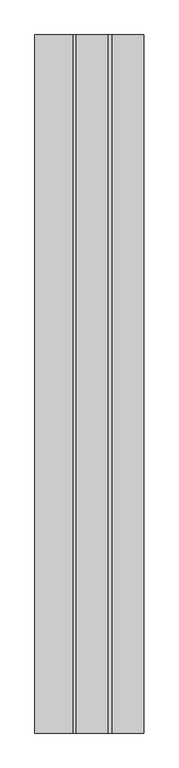
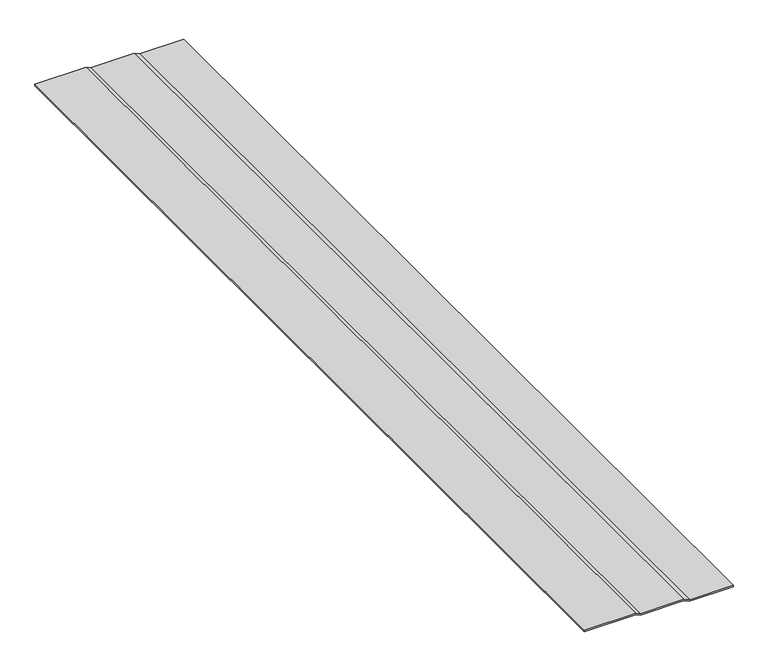
"""IFC4 building model written with IfcOpenShell, lengths in millimetres: proxy geometry, BITUMEN CAP SHEET001 3829 : BITUMEN CAP SHEET001 3829."""

from ifc_helpers import new_model, si_unit, frame, origin, place, context, project, spatial, polyline, outline, extrude, source, transform, mapped, element, save


def generic_models_3f8c56e2(model_context):
    return source(origin(), model_context, "Body", "SweptSolid", [
        extrude(outline(polyline([(40259.2002678, -4699.8063764), (40262.3752678, -4699.8063764), (40262.3752678, -4791.325638), (40267.6612773, -4803.7904566), (40267.6612773, -4894.4742123), (40271.9940719, -4904.1911138), (40271.9940719, -5012.0776104), (40268.8188423, -5012.0776104), (40268.8188423, -4904.8663993), (40264.4862773, -4895.1500128), (40264.4862773, -4804.4358566), (40259.2002678, -4791.971038), (40259.2002678, -4699.8063764)])), frame((0.0, -1052.8906574, 0.0), z_axis=(0.0, 1.0, 0.0), x_axis=(0.0, 0.0, 1.0)), (0.0, 0.0, 1.0), 2000.25),
    ])


if __name__ == "__main__":
    model = new_model("IFC4")
    model_context = context("Model", 3, world=origin())
    ifc_project = project(units=[si_unit("LENGTHUNIT", "METRE", prefix="MILLI")], contexts=[model_context])
    site = spatial("IfcSite", under=ifc_project)
    building = spatial("IfcBuilding", under=site)
    placement = place(None, origin())
    generic_models_shape = generic_models_3f8c56e2(model_context)
    element("IfcBuildingElementProxy", 1, Name="BITUMEN CAP SHEET001 3829 : BITUMEN CAP SHEET001 3829", ObjectType="BITUMEN CAP SHEET001 3829 : BITUMEN CAP SHEET001 3829", at=placement, inside=building, context=model_context, shape_type="MappedRepresentation", body=[
        mapped(generic_models_shape, transform((0.0, 0.0, 0.0), x_axis=(1.0, 0.0, 0.0), y_axis=(0.0, 1.0, 0.0), z_axis=(0.0, 0.0, 1.0))),
    ])
    save(model, "model.ifc")

# Revit data of these elements
# Type "BITUMEN CAP SHEET001 3829 : BITUMEN CAP SHEET001 3829"
#   NameOverride = "BITUMEN CAP SHEET001"
# Element 1 (IfcBuildingElementProxy, "BITUMEN CAP SHEET001 3829 : BITUMEN CAP SHEET001 3829")
#   Materials on its faces: "MODIFIED BITUMEN GRANULE SURFACED CAP SHEET"
# Materials
#   "MODIFIED BITUMEN GRANULE SURFACED CAP SHEET": class "Unassigned", colour RGB 85 85 127, transparency 0
